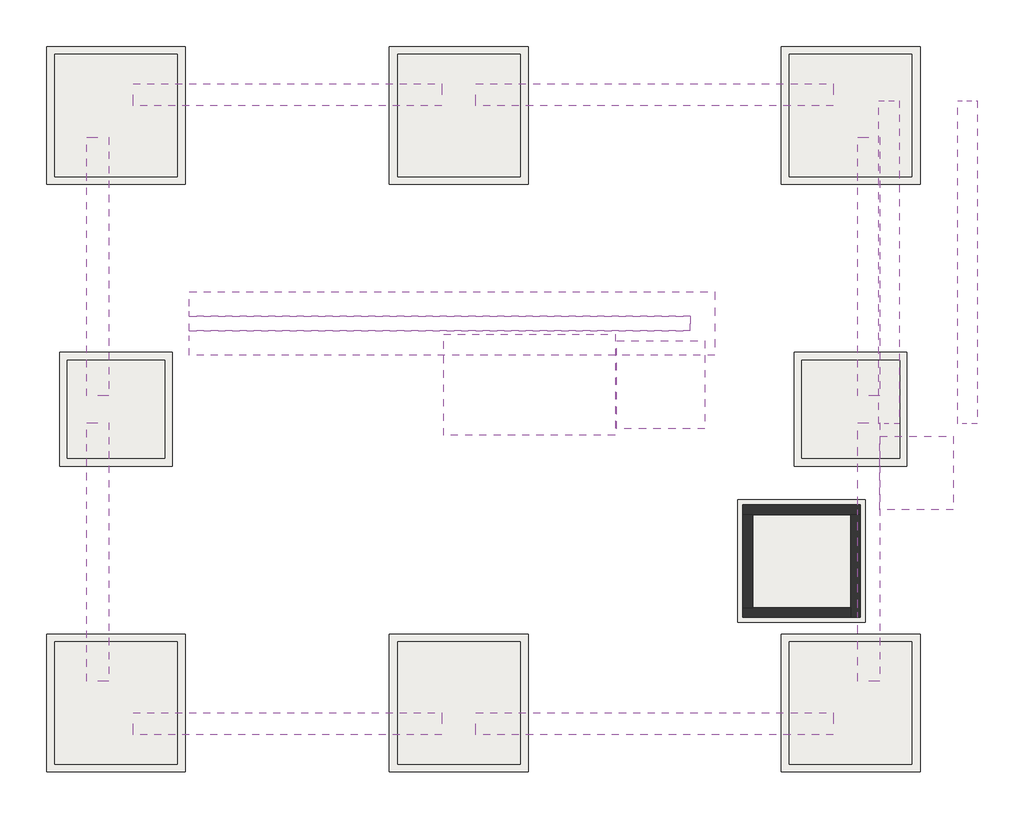
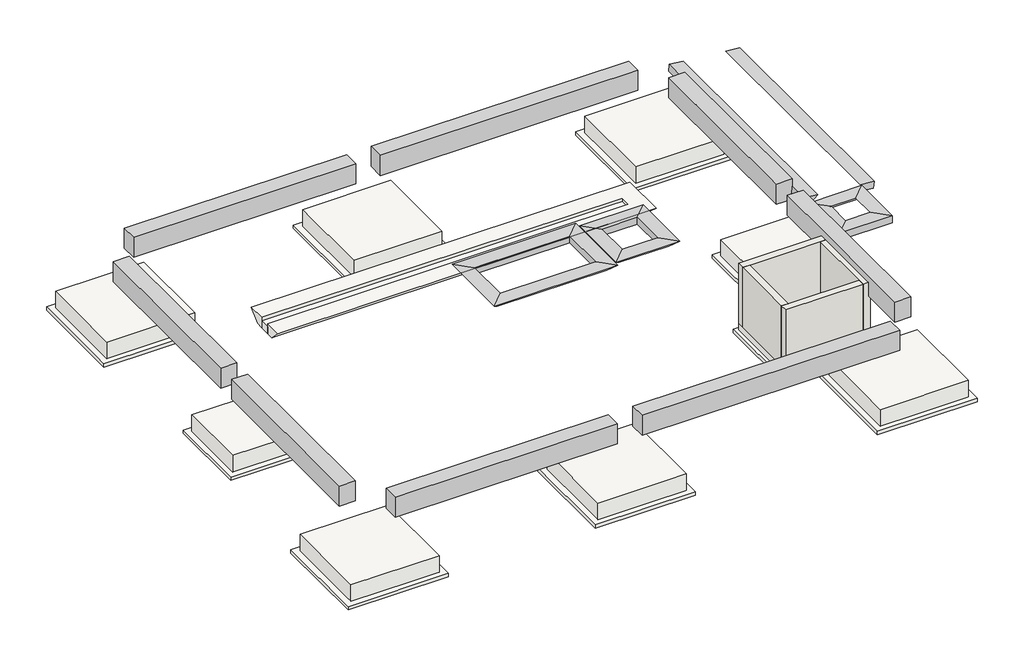
# One storey: 20 slabs, 7 beams, 5 proxies, 4 walls, 1 member.
"""IFC4 building model written with IfcOpenShell, lengths in millimetres."""

import ifcopenshell
import ifcopenshell.guid

model = None  # the IFC model being written
_history = None  # IfcOwnerHistory: only IFC2X3 demands one
_inside = {}  # id of a spatial element -> (the spatial element, [elements in it])
_under = {}  # id of a project, library or spatial element -> (it, [spatial elements below it])
_declared = {}  # id of a project -> (the project, [libraries it declares])
_typed = {}  # id of a type object -> (the type object, [elements of that type])
_made_of = {}  # id of a material, layer set ... -> (it, [elements and type objects made of it])


def new_model(schema):
    """Start an empty IFC model of exactly this schema.

    Asked for "IFC4X3", IfcOpenShell would pick the latest addendum, in which some entities
    have other attributes; the version numbers below select the first issue.
    IFC2X3 requires an IfcOwnerHistory on every rooted entity: one is made here for all.
    """
    global model, _history
    if schema == "IFC4X3":
        model = ifcopenshell.file(schema_version=(4, 3, 0, 0))
    else:
        model = ifcopenshell.file(schema=schema)
    _inside.clear()
    _under.clear()
    _declared.clear()
    _typed.clear()
    _made_of.clear()
    _history = None
    if model.schema == "IFC2X3":
        org = make("IfcOrganization", Name="unknown")
        user = make(
            "IfcPersonAndOrganization",
            ThePerson=make("IfcPerson", FamilyName="unknown"),
            TheOrganization=org,
        )
        app = make(
            "IfcApplication",
            ApplicationDeveloper=org,
            Version="unknown",
            ApplicationFullName="unknown",
            ApplicationIdentifier="unknown",
        )
        _history = make(
            "IfcOwnerHistory",
            OwningUser=user,
            OwningApplication=app,
            ChangeAction="ADDED",
            CreationDate=0,
        )
    return model


def make(cls, **values):
    """One entity of the class cls with the attributes given. An attribute that is None is left unset."""
    return model.create_entity(
        cls, **{name: value for name, value in values.items() if value is not None}
    )


def rooted(cls, **values):
    """An entity with a GlobalId (a new one), such as an element, a storey or a relation."""
    return make(cls, GlobalId=ifcopenshell.guid.new(), OwnerHistory=_history, **values)


def si_unit(unit_type, name, prefix=None):
    """IfcSIUnit, for example si_unit("LENGTHUNIT", "METRE", prefix="MILLI")."""
    return make("IfcSIUnit", UnitType=unit_type, Prefix=prefix, Name=name)


def assignment(units):
    """IfcUnitAssignment: the units of a project."""
    return None if units is None else make("IfcUnitAssignment", Units=units)


def point(xyz):
    """IfcCartesianPoint."""
    return None if xyz is None else make("IfcCartesianPoint", Coordinates=xyz)


def direction(xyz):
    """IfcDirection."""
    return None if xyz is None else make("IfcDirection", DirectionRatios=xyz)


def frame(location, z_axis=None, x_axis=None):
    """IfcAxis2Placement3D, a coordinate frame: its origin and axes. An axis left out is left unset."""
    return make(
        "IfcAxis2Placement3D",
        Location=point(location),
        Axis=direction(z_axis),
        RefDirection=direction(x_axis),
    )


def origin():
    """The frame at (0, 0, 0) with its axes left unset."""
    return frame((0.0, 0.0, 0.0))


def place(relative_to, where):
    """IfcLocalPlacement: puts the frame where relative to a parent placement (None: the world)."""
    return make(
        "IfcLocalPlacement", PlacementRelTo=relative_to, RelativePlacement=where
    )


def context(
    kind, dimensions, precision=None, world=None, true_north=None, identifier=None
):
    """IfcGeometricRepresentationContext, for example the 3D "Model" context."""
    return make(
        "IfcGeometricRepresentationContext",
        ContextIdentifier=identifier,
        ContextType=kind,
        CoordinateSpaceDimension=dimensions,
        Precision=precision,
        WorldCoordinateSystem=world,
        TrueNorth=true_north,
    )


def project(units=None, contexts=None):
    """IfcProject with its units and contexts."""
    return rooted(
        "IfcProject",
        Name="project",
        RepresentationContexts=contexts,
        UnitsInContext=assignment(units),
    )


def spatial(cls, under=None, at=None, **own):
    """A site, building, storey or space (cls), placed at a placement, below another one or the project."""
    s = rooted(cls, ObjectPlacement=at, **own)
    if under is not None:
        _under.setdefault(under.id(), (under, []))[1].append(s)
    return s


def polyline(points):
    """IfcPolyline through the points."""
    return make("IfcPolyline", Points=[point(p) for p in points])


def outline(outer, holes=None, kind="AREA"):
    """IfcArbitraryClosedProfileDef: a profile drawn as a closed curve; with holes, ...WithVoids."""
    if holes is None:
        return make("IfcArbitraryClosedProfileDef", ProfileType=kind, OuterCurve=outer)
    return make(
        "IfcArbitraryProfileDefWithVoids",
        ProfileType=kind,
        OuterCurve=outer,
        InnerCurves=holes,
    )


def extrude(swept, where, along, depth):
    """IfcExtrudedAreaSolid: the profile swept, set in the frame where, extruded along a direction by depth."""
    return make(
        "IfcExtrudedAreaSolid",
        SweptArea=swept,
        Position=where,
        ExtrudedDirection=direction(along),
        Depth=depth,
    )


def faces_of(points, faces, orient=None, outer=None):
    """IfcFace entities. A face is a list of loops; a loop is a list of indices into points, from 0.

    orient and outer hold one flag for each loop. By default every Orientation is true, the
    first loop of a face is its IfcFaceOuterBound and the others are IfcFaceBound.
    """
    made = []
    for i, loops in enumerate(faces):
        bounds = []
        for j, loop in enumerate(loops):
            is_outer = j == 0 if outer is None else outer[i][j]
            bounds.append(
                make(
                    "IfcFaceOuterBound" if is_outer else "IfcFaceBound",
                    Bound=make("IfcPolyLoop", Polygon=[points[k] for k in loop]),
                    Orientation=True if orient is None else orient[i][j],
                )
            )
        made.append(make("IfcFace", Bounds=bounds))
    return made


def faceted_brep(points, faces, orient=None, outer=None, voids=None):
    """IfcFacetedBrep: a solid bounded by flat faces; with voids (closed shells), ...WithVoids."""
    shared = [point(p) for p in points]
    hull = make("IfcClosedShell", CfsFaces=faces_of(shared, faces, orient, outer))
    if voids is None:
        return make("IfcFacetedBrep", Outer=hull)
    return make(
        "IfcFacetedBrepWithVoids",
        Outer=hull,
        Voids=[
            make(cls, CfsFaces=faces_of(shared, fs, o, b)) for cls, fs, o, b in voids
        ],
    )


def shape(context_of_items, identifier, shape_type, items):
    """IfcShapeRepresentation: the items that make up one representation, for example the "Body"."""
    return make(
        "IfcShapeRepresentation",
        ContextOfItems=context_of_items,
        RepresentationIdentifier=identifier,
        RepresentationType=shape_type,
        Items=items,
    )


def source(mapping_origin, context_of_items, identifier, shape_type, items):
    """IfcRepresentationMap: a shape defined once, which mapped items show again and again."""
    return make(
        "IfcRepresentationMap",
        MappingOrigin=mapping_origin,
        MappedRepresentation=shape(context_of_items, identifier, shape_type, items),
    )


def transform(
    local_origin,
    x_axis=None,
    y_axis=None,
    z_axis=None,
    scale=None,
    scale2=None,
    scale3=None,
    uniform=True,
):
    """IfcCartesianTransformationOperator3D, or its non-uniform kind. x_axis, y_axis, z_axis: its Axis1, 2, 3."""
    if uniform:
        return make(
            "IfcCartesianTransformationOperator3D",
            Axis1=direction(x_axis),
            Axis2=direction(y_axis),
            LocalOrigin=point(local_origin),
            Scale=scale,
            Axis3=direction(z_axis),
        )
    return make(
        "IfcCartesianTransformationOperator3DnonUniform",
        Axis1=direction(x_axis),
        Axis2=direction(y_axis),
        LocalOrigin=point(local_origin),
        Scale=scale,
        Axis3=direction(z_axis),
        Scale2=scale2,
        Scale3=scale3,
    )


def mapped(mapping_source, mapping_target):
    """IfcMappedItem: shows the shape of a source again, moved by a transform."""
    return make(
        "IfcMappedItem", MappingSource=mapping_source, MappingTarget=mapping_target
    )


def made_of(thing, what):
    """Note that an element or type object is made of a material, layer set ...; save() writes the relation."""
    if what is not None:
        _made_of.setdefault(what.id(), (what, []))[1].append(thing)
    return thing


def element(
    cls,
    number,
    at=None,
    inside=None,
    cuts=None,
    type_object=None,
    material=None,
    context=None,
    identifier="Body",
    shape_type=None,
    held_by="IfcProductDefinitionShape",
    body=None,
    shapes=None,
    **own,
):
    """One element of the class cls, such as IfcWall. Its Tag is "e" and its number.

    at: its placement. inside: the storey or other place that contains it. cuts: it is an
    opening in that element (IfcRelVoidsElement). A single representation is given by context,
    identifier, shape_type and body (its items); several are given by shapes. held_by: the class
    of the entity that holds the representations. save() writes the other relations.
    """
    e = rooted(cls, Tag="e%d" % number, ObjectPlacement=at, **own)
    if body is not None:
        shapes = [shape(context, identifier, shape_type, body)]
    if shapes is not None:
        e.Representation = make(held_by, Representations=shapes)
    if inside is not None:
        _inside.setdefault(inside.id(), (inside, []))[1].append(e)
    if cuts is not None:
        rooted(
            "IfcRelVoidsElement", RelatingBuildingElement=cuts, RelatedOpeningElement=e
        )
    if type_object is not None:
        _typed.setdefault(type_object.id(), (type_object, []))[1].append(e)
    return made_of(e, material)


def aggregate(whole, parts):
    """IfcRelAggregates: a whole, such as a stair, and the parts it consists of."""
    return rooted("IfcRelAggregates", RelatingObject=whole, RelatedObjects=parts)


def save(model, path):
    """Write the relations noted so far, then the file.

    IfcRelAggregates (storeys below a building ...), IfcRelContainedInSpatialStructure (elements
    in a storey), IfcRelDefinesByType, IfcRelAssociatesMaterial and IfcRelDeclares: one each for
    every whole, place, type object, material and project.
    """
    for whole, parts in _under.values():
        aggregate(whole, parts)
    for where, things in _inside.values():
        rooted(
            "IfcRelContainedInSpatialStructure",
            RelatedElements=things,
            RelatingStructure=where,
        )
    for kind, things in _typed.values():
        rooted("IfcRelDefinesByType", RelatedObjects=things, RelatingType=kind)
    for what, things in _made_of.values():
        rooted("IfcRelAssociatesMaterial", RelatedObjects=things, RelatingMaterial=what)
    for by, libraries in _declared.values():
        rooted("IfcRelDeclares", RelatingContext=by, RelatedDefinitions=libraries)
    model.write(path)


def slab_cd841ba3(model_context):
    return source(origin(), model_context, "Body", "Brep", [
        faceted_brep([(100.0, 18494.5382614, -200.0), (100.0, 18994.5382614, -200.0), (100.0, 18694.5382614, -500.0), (100.0, 18494.5382614, -500.0), (100.0, 18494.5382614, -300.0), (10325.0, 18494.5382614, -500.0), (10325.0, 18494.5382614, -300.0), (10325.0, 18494.5382614, -200.0), (10325.0, 18194.5382614, -200.0), (100.0, 18194.5382614, -200.0), (100.0, 17694.5382614, -200.0), (10825.0, 17694.5382614, -200.0), (10825.0, 18994.5382614, -200.0), (10525.0, 18694.5382614, -500.0), (10525.0, 17994.5382614, -500.0), (100.0, 17994.5382614, -500.0), (100.0, 18194.5382614, -500.0), (10325.0, 18194.5382614, -500.0), (10325.0, 18194.5382614, -300.0), (100.0, 18194.5382614, -300.0)], [[[0, 1, 2, 3, 4]], [[3, 5, 6, 7, 0, 4]], [[1, 0, 7, 8, 9, 10, 11, 12]], [[2, 1, 12, 13]], [[3, 2, 13, 14, 15, 16, 17, 5]], [[8, 7, 6, 5, 17, 18]], [[13, 12, 11, 14]], [[10, 9, 19, 16, 15]], [[9, 8, 18, 17, 16, 19]], [[15, 14, 11, 10]]]),
    ])


def slab_e6aba4ee(model_context):
    return source(origin(), model_context, "Body", "SweptSolid", [
        extrude(outline(polyline([(100.0, 18194.5382614), (100.0, 18494.5382614), (10325.0, 18494.5382614), (10325.0, 18194.5382614), (100.0, 18194.5382614)])), frame((0.0, 0.0, -500.0), z_axis=(0.0, 0.0, 1.0), x_axis=(1.0, 0.0, 0.0)), (0.0, 0.0, 1.0), 200.0),
    ])


def ft112_footing_rectangular_ft112_2000x2000x500_8ee35437(model_context):
    return source(origin(), model_context, "Body", "SweptSolid", [
        extrude(outline(polyline([(1000.0, 1000.0), (1000.0, -1000.0), (-1000.0, -1000.0), (-1000.0, 1000.0), (1000.0, 1000.0)])), frame((0.0, 0.0, -500.0), z_axis=(0.0, 0.0, 1.0), x_axis=(1.0, 0.0, 0.0)), (0.0, 0.0, 1.0), 500.0),
    ])


def ft112_footing_rectangular_ft112_2500x2500x500_513089b3(model_context):
    return source(origin(), model_context, "Body", "SweptSolid", [
        extrude(outline(polyline([(1250.0, 1250.0), (1250.0, -1250.0), (-1250.0, -1250.0), (-1250.0, 1250.0), (1250.0, 1250.0)])), frame((0.0, 0.0, -500.0), z_axis=(0.0, 0.0, 1.0), x_axis=(1.0, 0.0, 0.0)), (0.0, 0.0, 1.0), 500.0),
    ])


model = new_model("IFC4")

# Units and contexts
model_context = context("Model", 3, world=origin())
ifc_project = project(units=[si_unit("LENGTHUNIT", "METRE", prefix="MILLI")], contexts=[model_context])

# Site, building, storey
site = spatial("IfcSite", under=ifc_project)
building = spatial("IfcBuilding", under=site)
storey = spatial("IfcBuildingStorey", under=building, Name="1.B.O.F (FL -2200)", Elevation=-2200.0)

# Beams
placement = place(None, origin())
element("IfcBeam", 1, ObjectType="Concrete-Rectangular-Beam : BM112_450x600_UG", at=placement, inside=storey, context=model_context, shape_type="Brep", body=[
    faceted_brep([(13250.0, 9944.5382614, 0.0), (13250.0, 10394.5382614, 0.0), (5950.0, 10394.5382614, 0.0), (5950.0, 9944.5382614, 0.0), (13250.0, 9944.5382614, -600.0), (5950.0, 9944.5382614, -600.0), (13250.0, 10394.5382614, -600.0), (5950.0, 10394.5382614, -600.0), (13250.0, 10394.5382614, -200.0), (5950.0, 10394.5382614, -200.0)], [[[0, 1, 2, 3]], [[4, 0, 3, 5]], [[6, 4, 5, 7]], [[1, 8, 6, 7, 9, 2]], [[2, 9, 7, 5, 3]], [[1, 0, 4, 6, 8]]]),
])
element("IfcBeam", 2, ObjectType="Concrete-Rectangular-Beam : BM112_450x600_UG", at=placement, inside=storey, context=model_context, shape_type="Brep", body=[
    faceted_brep([(13750.0, 16319.5382614, 0.0), (13750.0, 14444.5382614, 0.0), (13750.0, 12544.5382614, 0.0), (13750.0, 11044.5382614, 0.0), (14200.0, 11044.5382614, 0.0), (14200.0, 16319.5382614, 0.0), (14200.0, 11044.5382614, -600.0), (14200.0, 16319.5382614, -600.0), (13750.0, 11044.5382614, -600.0), (13750.0, 12344.5382614, -600.0), (13800.0, 12344.5382614, -600.0), (13800.0, 14644.5382614, -600.0), (13750.0, 14644.5382614, -600.0), (13750.0, 16319.5382614, -600.0), (13750.0, 16319.5382614, -200.0), (13750.0, 14644.5382614, -200.0), (13750.0, 14444.5382614, -200.0), (13750.0, 12544.5382614, -200.0), (13750.0, 12344.5382614, -200.0), (13750.0, 11044.5382614, -200.0), (13800.0, 14644.5382614, -200.0), (13800.0, 12344.5382614, -200.0), (13800.0, 14444.5382614, -200.0)], [[[0, 1, 2, 3, 4, 5]], [[5, 4, 6, 7]], [[7, 6, 8, 9, 10, 11, 12, 13]], [[3, 2, 1, 0, 14, 13, 12, 15, 16, 17, 18, 9, 8, 19]], [[11, 20, 15, 12]], [[21, 18, 17, 16, 15, 20, 22]], [[21, 22, 20, 11, 10]], [[21, 10, 9, 18]], [[3, 19, 8, 6, 4]], [[0, 5, 7, 13, 14]]]),
])
element("IfcBeam", 3, ObjectType="Concrete-Rectangular-Beam : BM112_450x600_UG", at=placement, inside=storey, context=model_context, shape_type="Brep", body=[
    faceted_brep([(14200.0, 22144.5382614, 0.0), (13750.0, 22144.5382614, 0.0), (13750.0, 16869.5382614, 0.0), (14200.0, 16869.5382614, 0.0), (14200.0, 22144.5382614, -600.0), (14200.0, 16869.5382614, -600.0), (13750.0, 22144.5382614, -600.0), (13750.0, 16869.5382614, -600.0), (13750.0, 22144.5382614, -200.0), (13750.0, 16869.5382614, -200.0)], [[[0, 1, 2, 3]], [[4, 0, 3, 5]], [[6, 4, 5, 7]], [[1, 8, 6, 7, 9, 2]], [[1, 0, 4, 6, 8]], [[3, 2, 9, 7, 5]]]),
])
element("IfcBeam", 4, ObjectType="Concrete-Rectangular-Beam : BM112_450x600_UG", at=placement, inside=storey, context=model_context, shape_type="Brep", body=[
    faceted_brep([(5950.0, 23244.5382614, 0.0), (5950.0, 22794.5382614, 0.0), (13250.0, 22794.5382614, 0.0), (13250.0, 23244.5382614, 0.0), (5950.0, 23244.5382614, -600.0), (13250.0, 23244.5382614, -600.0), (5950.0, 22794.5382614, -600.0), (13250.0, 22794.5382614, -600.0), (5950.0, 22794.5382614, -200.0), (13250.0, 22794.5382614, -200.0)], [[[0, 1, 2, 3]], [[4, 0, 3, 5]], [[6, 4, 5, 7]], [[1, 8, 6, 7, 9, 2]], [[1, 0, 4, 6, 8]], [[3, 2, 9, 7, 5]]]),
])
element("IfcBeam", 5, ObjectType="Concrete-Rectangular-Beam : BM112_450x600_UG", at=placement, inside=storey, context=model_context, shape_type="Brep", body=[
    faceted_brep([(5250.0, 22794.5382614, 0.0), (5250.0, 23244.5382614, 0.0), (-1050.0, 23244.5382614, 0.0), (-1050.0, 22794.5382614, 0.0), (5250.0, 23244.5382614, -600.0), (-1050.0, 23244.5382614, -600.0), (5250.0, 22794.5382614, -600.0), (-1050.0, 22794.5382614, -600.0), (5250.0, 22794.5382614, -200.0), (-1050.0, 22794.5382614, -200.0)], [[[0, 1, 2, 3]], [[1, 4, 5, 2]], [[4, 6, 7, 5]], [[6, 8, 0, 3, 9, 7]], [[1, 0, 8, 6, 4]], [[3, 2, 5, 7, 9]]]),
])
element("IfcBeam", 6, ObjectType="Concrete-Rectangular-Beam : BM112_450x600_UG", at=placement, inside=storey, context=model_context, shape_type="Brep", body=[
    faceted_brep([(-1550.0, 22144.5382614, 0.0), (-2000.0, 22144.5382614, 0.0), (-2000.0, 16869.5382614, 0.0), (-1550.0, 16869.5382614, 0.0), (-2000.0, 22144.5382614, -600.0), (-2000.0, 16869.5382614, -600.0), (-1550.0, 22144.5382614, -600.0), (-1550.0, 16869.5382614, -600.0), (-1550.0, 22144.5382614, -200.0), (-1550.0, 16869.5382614, -200.0)], [[[0, 1, 2, 3]], [[1, 4, 5, 2]], [[4, 6, 7, 5]], [[6, 8, 0, 3, 9, 7]], [[1, 0, 8, 6, 4]], [[3, 2, 5, 7, 9]]]),
])
element("IfcBeam", 7, ObjectType="Concrete-Rectangular-Beam : BM112_450x600_UG", at=placement, inside=storey, context=model_context, shape_type="Brep", body=[
    faceted_brep([(-2000.0, 11044.5382614, 0.0), (-1550.0, 11044.5382614, 0.0), (-1550.0, 16319.5382614, 0.0), (-2000.0, 16319.5382614, 0.0), (-2000.0, 11044.5382614, -600.0), (-2000.0, 16319.5382614, -600.0), (-1550.0, 11044.5382614, -600.0), (-1550.0, 16319.5382614, -600.0), (-1550.0, 11044.5382614, -200.0), (-1550.0, 16319.5382614, -200.0)], [[[0, 1, 2, 3]], [[4, 0, 3, 5]], [[6, 4, 5, 7]], [[1, 8, 6, 7, 9, 2]], [[1, 0, 4, 6, 8]], [[3, 2, 9, 7, 5]]]),
])

# Proxies
element("IfcBuildingElementProxy", 8, Name="Slab Edge", ObjectType="Slab Edge", at=placement, inside=storey, context=model_context, shape_type="Brep", body=[
    faceted_brep([(8390.0, 16459.5382614, -200.0), (8390.0, 16459.5382614, -400.0), (5690.0, 16459.5382614, -400.0), (5690.0, 16459.5382614, -200.0), (8790.0, 16059.5382614, -200.0), (5290.0, 16059.5382614, -200.0), (8590.0, 16259.5382614, -400.0), (5490.0, 16259.5382614, -400.0), (8390.0, 17729.5382614, -200.0), (8390.0, 17729.5382614, -400.0), (8790.0, 18129.5382614, -200.0), (8590.0, 17929.5382614, -400.0), (5690.0, 17729.5382614, -200.0), (5690.0, 17729.5382614, -400.0), (5290.0, 18129.5382614, -200.0), (5490.0, 17929.5382614, -400.0)], [[[0, 1, 2, 3]], [[4, 0, 3, 5]], [[6, 4, 5, 7]], [[1, 6, 7, 2]], [[8, 9, 1, 0]], [[10, 8, 0, 4]], [[11, 10, 4, 6]], [[9, 11, 6, 1]], [[12, 13, 9, 8]], [[14, 12, 8, 10]], [[15, 14, 10, 11]], [[13, 15, 11, 9]], [[3, 2, 13, 12]], [[5, 3, 12, 14]], [[7, 5, 14, 15]], [[2, 7, 15, 13]]]),
])
element("IfcBuildingElementProxy", 9, Name="Slab Edge", ObjectType="Slab Edge", at=placement, inside=storey, context=model_context, shape_type="Brep", body=[
    faceted_brep([(10225.0, 16594.5382614, -200.0), (10225.0, 16594.5382614, -400.0), (9225.0, 16594.5382614, -400.0), (9225.0, 16594.5382614, -200.0), (10625.0, 16194.5382614, -200.0), (8825.0, 16194.5382614, -200.0), (10425.0, 16394.5382614, -400.0), (9025.0, 16394.5382614, -400.0), (10225.0, 17594.5382614, -200.0), (10225.0, 17594.5382614, -400.0), (10625.0, 17994.5382614, -200.0), (10425.0, 17794.5382614, -400.0), (9225.0, 17594.5382614, -200.0), (9225.0, 17594.5382614, -400.0), (8825.0, 17994.5382614, -200.0), (9025.0, 17794.5382614, -400.0)], [[[0, 1, 2, 3]], [[4, 0, 3, 5]], [[6, 4, 5, 7]], [[1, 6, 7, 2]], [[8, 9, 1, 0]], [[10, 8, 0, 4]], [[11, 10, 4, 6]], [[9, 11, 6, 1]], [[12, 13, 9, 8]], [[14, 12, 8, 10]], [[15, 14, 10, 11]], [[13, 15, 11, 9]], [[3, 2, 13, 12]], [[5, 3, 12, 14]], [[7, 5, 14, 15]], [[2, 7, 15, 13]]]),
])
element("IfcBuildingElementProxy", 10, Name="Slab Edge", ObjectType="Slab Edge", at=placement, inside=storey, context=model_context, shape_type="SweptSolid", body=[
    extrude(outline(polyline([(-620.0141724, 16171.1013164), (-421.0065284, 16191.0), (-381.2091611, 15792.9847119), (-600.1154888, 15972.0936723), (-620.0141724, 16171.1013164)])), frame((0.0, 16294.5382614, 0.0), z_axis=(0.0, 1.0, 0.0), x_axis=(0.0, 0.0, 1.0)), (0.0, 0.0, 1.0), 6600.0),
])
element("IfcBuildingElementProxy", 11, Name="Slab Edge", ObjectType="Slab Edge", at=placement, inside=storey, context=model_context, shape_type="SweptSolid", body=[
    extrude(outline(polyline([(-420.0141724, 14180.1013164), (-439.9128561, 14379.1089604), (-260.8038956, 14598.0152881), (-221.0065284, 14200.0), (-420.0141724, 14180.1013164)])), frame((0.0, 16294.5382614, 0.0), z_axis=(0.0, 1.0, 0.0), x_axis=(0.0, 0.0, 1.0)), (0.0, 0.0, 1.0), 6600.0),
])
element("IfcBuildingElementProxy", 12, Name="Slab Edge", ObjectType="Slab Edge", at=placement, inside=storey, context=model_context, shape_type="Brep", body=[
    faceted_brep([(14200.0, 16044.5382614, -220.0), (14200.0, 16044.5382614, -420.0), (14200.0, 14544.5382614, -420.0), (14200.0, 14544.5382614, -220.0), (14600.0, 15644.5382614, -220.0), (14600.0, 14944.5382614, -220.0), (14400.0, 15844.5382614, -420.0), (14400.0, 14744.5382614, -420.0), (15700.0, 14544.5382614, -420.0), (15700.0, 14544.5382614, -220.0), (15300.0, 14944.5382614, -220.0), (15500.0, 14744.5382614, -420.0), (15700.0, 16044.5382614, -420.0), (15700.0, 16044.5382614, -220.0), (15300.0, 15644.5382614, -220.0), (15500.0, 15844.5382614, -420.0)], [[[0, 1, 2, 3]], [[4, 0, 3, 5]], [[6, 4, 5, 7]], [[1, 6, 7, 2]], [[3, 2, 8, 9]], [[5, 3, 9, 10]], [[7, 5, 10, 11]], [[2, 7, 11, 8]], [[9, 8, 12, 13]], [[10, 9, 13, 14]], [[11, 10, 14, 15]], [[8, 11, 15, 12]], [[13, 12, 1, 0]], [[14, 13, 0, 4]], [[15, 14, 4, 6]], [[12, 15, 6, 1]]]),
])

# Member
element("IfcMember", 13, ObjectType="Concrete-Rectangular-Beam : BM112_450x600_UG", at=placement, inside=storey, context=model_context, shape_type="Brep", body=[
    faceted_brep([(5250.0, 9944.5382614, 0.0), (5250.0, 10394.5382614, 0.0), (-1050.0, 10394.5382614, 0.0), (-1050.0, 9944.5382614, 0.0), (5250.0, 9944.5382614, -600.0), (-1050.0, 9944.5382614, -600.0), (5250.0, 10394.5382614, -600.0), (-1050.0, 10394.5382614, -600.0), (5250.0, 10394.5382614, -200.0), (-1050.0, 10394.5382614, -200.0)], [[[0, 1, 2, 3]], [[4, 0, 3, 5]], [[6, 4, 5, 7]], [[1, 8, 6, 7, 9, 2]], [[2, 9, 7, 5, 3]], [[1, 0, 4, 6, 8]]]),
])

# Slabs
element("IfcSlab", 14, ObjectType="SL101_Lean Floor_100", at=placement, inside=storey, context=model_context, shape_type="SweptSolid", body=[
    extrude(outline(polyline([(18.583556, 12001.1722664), (18.583556, 9187.9042565), (-2818.583556, 9187.9042565), (-2818.583556, 12001.1722664), (18.583556, 12001.1722664)])), frame((0.0, 0.0, -2300.0), z_axis=(0.0, 0.0, 1.0), x_axis=(1.0, 0.0, 0.0)), (0.0, 0.0, 1.0), 100.0),
])
element("IfcSlab", 15, ObjectType="SL101_Lean Floor_100", at=placement, inside=storey, context=model_context, shape_type="SweptSolid", body=[
    extrude(outline(polyline([(7018.583556, 12001.1722664), (7018.583556, 9187.9042565), (4181.416444, 9187.9042565), (4181.416444, 12001.1722664), (7018.583556, 12001.1722664)])), frame((0.0, 0.0, -2300.0), z_axis=(0.0, 0.0, 1.0), x_axis=(1.0, 0.0, 0.0)), (0.0, 0.0, 1.0), 100.0),
])
element("IfcSlab", 16, ObjectType="SL101_Lean Floor_100", at=placement, inside=storey, context=model_context, shape_type="SweptSolid", body=[
    extrude(outline(polyline([(15018.583556, 12001.1722664), (15018.583556, 9187.9042565), (12181.416444, 9187.9042565), (12181.416444, 12001.1722664), (15018.583556, 12001.1722664)])), frame((0.0, 0.0, -2300.0), z_axis=(0.0, 0.0, 1.0), x_axis=(1.0, 0.0, 0.0)), (0.0, 0.0, 1.0), 100.0),
])
element("IfcSlab", 17, ObjectType="SL101_Lean Floor_100", at=placement, inside=storey, context=model_context, shape_type="SweptSolid", body=[
    extrude(outline(polyline([(18.583556, 24001.1722664), (18.583556, 21187.9042565), (-2818.583556, 21187.9042565), (-2818.583556, 24001.1722664), (18.583556, 24001.1722664)])), frame((0.0, 0.0, -2300.0), z_axis=(0.0, 0.0, 1.0), x_axis=(1.0, 0.0, 0.0)), (0.0, 0.0, 1.0), 100.0),
])
element("IfcSlab", 18, ObjectType="SL101_Lean Floor_100", at=placement, inside=storey, context=model_context, shape_type="SweptSolid", body=[
    extrude(outline(polyline([(7018.583556, 24001.1722664), (7018.583556, 21187.9042565), (4181.416444, 21187.9042565), (4181.416444, 24001.1722664), (7018.583556, 24001.1722664)])), frame((0.0, 0.0, -2300.0), z_axis=(0.0, 0.0, 1.0), x_axis=(1.0, 0.0, 0.0)), (0.0, 0.0, 1.0), 100.0),
])
element("IfcSlab", 19, ObjectType="SL101_Lean Floor_100", at=placement, inside=storey, context=model_context, shape_type="SweptSolid", body=[
    extrude(outline(polyline([(15018.583556, 24001.1722664), (15018.583556, 21187.9042565), (12181.416444, 21187.9042565), (12181.416444, 24001.1722664), (15018.583556, 24001.1722664)])), frame((0.0, 0.0, -2300.0), z_axis=(0.0, 0.0, 1.0), x_axis=(1.0, 0.0, 0.0)), (0.0, 0.0, 1.0), 100.0),
])
element("IfcSlab", 20, ObjectType="SL101_Lean Floor_100", at=placement, inside=storey, context=model_context, shape_type="SweptSolid", body=[
    extrude(outline(polyline([(-251.1867019, 17756.5623227), (-251.1867019, 15432.5142002), (-2548.8132981, 15432.5142002), (-2548.8132981, 17756.5623227), (-251.1867019, 17756.5623227)])), frame((0.0, 0.0, -2300.0), z_axis=(0.0, 0.0, 1.0), x_axis=(1.0, 0.0, 0.0)), (0.0, 0.0, 1.0), 100.0),
])
element("IfcSlab", 21, ObjectType="SL101_Lean Floor_100", at=placement, inside=storey, context=model_context, shape_type="SweptSolid", body=[
    extrude(outline(polyline([(14748.8132981, 17756.5623227), (14748.8132981, 15432.5142002), (12451.1867019, 15432.5142002), (12451.1867019, 17756.5623227), (14748.8132981, 17756.5623227)])), frame((0.0, 0.0, -2300.0), z_axis=(0.0, 0.0, 1.0), x_axis=(1.0, 0.0, 0.0)), (0.0, 0.0, 1.0), 100.0),
])
element("IfcSlab", 22, ObjectType="SL101_Lean Floor_100", at=placement, inside=storey, context=model_context, shape_type="SweptSolid", body=[
    extrude(outline(polyline([(13900.0, 14744.5382614), (13900.0, 12244.5382614), (11300.0, 12244.5382614), (11300.0, 14744.5382614), (13900.0, 14744.5382614)])), frame((0.0, 0.0, -2300.0), z_axis=(0.0, 0.0, 1.0), x_axis=(1.0, 0.0, 0.0)), (0.0, 0.0, 1.0), 100.0),
])
slab_shape = slab_cd841ba3(model_context)
element("IfcSlab", 23, ObjectType="Ditch Wall 1 : Ditch Wall 1", at=placement, inside=storey, context=model_context, shape_type="MappedRepresentation", body=[
    mapped(slab_shape, transform((0.0, 0.0, 0.0), x_axis=(1.0, 0.0, 0.0), y_axis=(0.0, 1.0, 0.0), z_axis=(0.0, 0.0, 1.0))),
])
slab_2_shape = slab_e6aba4ee(model_context)
element("IfcSlab", 24, ObjectType="Ditch 2 : Ditch 2", at=placement, inside=storey, context=model_context, shape_type="MappedRepresentation", body=[
    mapped(slab_2_shape, transform((0.0, 0.0, 0.0), x_axis=(1.0, 0.0, 0.0), y_axis=(0.0, 1.0, 0.0), z_axis=(0.0, 0.0, 1.0))),
])
ft112_footing_rectangular_ft112_2000x2000x500_shape = ft112_footing_rectangular_ft112_2000x2000x500_8ee35437(model_context)
element("IfcSlab", 25, ObjectType="FT112-Footing-Rectangular : FT112_2000x2000x500", at=placement, inside=storey, context=model_context, shape_type="MappedRepresentation", body=[
    mapped(ft112_footing_rectangular_ft112_2000x2000x500_shape, transform((-1400.0, 16594.5382614, -1700.0), x_axis=(1.0, 0.0, 0.0), y_axis=(0.0, 1.0, 0.0), z_axis=(0.0, 0.0, 1.0))),
])
element("IfcSlab", 26, ObjectType="FT112-Footing-Rectangular : FT112_2000x2000x500", at=placement, inside=storey, context=model_context, shape_type="MappedRepresentation", body=[
    mapped(ft112_footing_rectangular_ft112_2000x2000x500_shape, transform((13600.0, 16594.5382614, -1700.0), x_axis=(1.0, 0.0, 0.0), y_axis=(0.0, 1.0, 0.0), z_axis=(0.0, 0.0, 1.0))),
])
element("IfcSlab", 27, ObjectType="FT112-Footing-Rectangular : FT112_2500x2500x500", at=placement, inside=storey, context=model_context, shape_type="SweptSolid", body=[
    extrude(outline(polyline([(-150.0, 11844.5382614), (-150.0, 9344.5382614), (-2650.0, 9344.5382614), (-2650.0, 11844.5382614), (-150.0, 11844.5382614)])), frame((0.0, 0.0, -2200.0), z_axis=(0.0, 0.0, 1.0), x_axis=(1.0, 0.0, 0.0)), (0.0, 0.0, 1.0), 500.0),
])
ft112_footing_rectangular_ft112_2500x2500x500_shape = ft112_footing_rectangular_ft112_2500x2500x500_513089b3(model_context)
element("IfcSlab", 28, ObjectType="FT112-Footing-Rectangular : FT112_2500x2500x500", at=placement, inside=storey, context=model_context, shape_type="MappedRepresentation", body=[
    mapped(ft112_footing_rectangular_ft112_2500x2500x500_shape, transform((-1400.0, 22594.5382614, -1700.0), x_axis=(1.0, 0.0, 0.0), y_axis=(0.0, 1.0, 0.0), z_axis=(0.0, 0.0, 1.0))),
])
element("IfcSlab", 29, ObjectType="FT112-Footing-Rectangular : FT112_2500x2500x500", at=placement, inside=storey, context=model_context, shape_type="MappedRepresentation", body=[
    mapped(ft112_footing_rectangular_ft112_2500x2500x500_shape, transform((5600.0, 22594.5382614, -1700.0), x_axis=(1.0, 0.0, 0.0), y_axis=(0.0, 1.0, 0.0), z_axis=(0.0, 0.0, 1.0))),
])
element("IfcSlab", 30, ObjectType="FT112-Footing-Rectangular : FT112_2500x2500x500", at=placement, inside=storey, context=model_context, shape_type="MappedRepresentation", body=[
    mapped(ft112_footing_rectangular_ft112_2500x2500x500_shape, transform((13600.0, 22594.5382614, -1700.0), x_axis=(1.0, 0.0, 0.0), y_axis=(0.0, 1.0, 0.0), z_axis=(0.0, 0.0, 1.0))),
])
element("IfcSlab", 31, ObjectType="FT112-Footing-Rectangular : FT112_2500x2500x500", at=placement, inside=storey, context=model_context, shape_type="MappedRepresentation", body=[
    mapped(ft112_footing_rectangular_ft112_2500x2500x500_shape, transform((13600.0, 10594.5382614, -1700.0), x_axis=(1.0, 0.0, 0.0), y_axis=(0.0, 1.0, 0.0), z_axis=(0.0, 0.0, 1.0))),
])
element("IfcSlab", 32, ObjectType="FT112-Footing-Rectangular : FT112_2500x2500x500", at=placement, inside=storey, context=model_context, shape_type="MappedRepresentation", body=[
    mapped(ft112_footing_rectangular_ft112_2500x2500x500_shape, transform((5600.0, 10594.5382614, -1700.0), x_axis=(1.0, 0.0, 0.0), y_axis=(0.0, 1.0, 0.0), z_axis=(0.0, 0.0, 1.0))),
])
element("IfcSlab", 33, ObjectType="MF111_THK.200", at=placement, inside=storey, context=model_context, shape_type="SweptSolid", body=[
    extrude(outline(polyline([(13800.0, 14644.5382614), (13800.0, 12344.5382614), (11400.0, 12344.5382614), (11400.0, 14644.5382614), (13800.0, 14644.5382614)])), frame((0.0, 0.0, -2200.0), z_axis=(0.0, 0.0, 1.0), x_axis=(1.0, 0.0, 0.0)), (0.0, 0.0, 1.0), 200.0),
])

# Walls
element("IfcWall", 34, ObjectType="WA111-UG RC Wall 200mm", at=placement, inside=storey, context=model_context, shape_type="Brep", body=[
    faceted_brep([(11400.0, 14444.5382614, -2000.0), (11600.0, 14444.5382614, -2000.0), (13600.0, 14444.5382614, -2000.0), (13800.0, 14444.5382614, -2000.0), (13800.0, 14444.5382614, -200.0), (13600.0, 14444.5382614, -200.0), (11600.0, 14444.5382614, -200.0), (11400.0, 14444.5382614, -200.0), (11400.0, 14644.5382614, -2000.0), (11400.0, 14644.5382614, -200.0), (13750.0, 14644.5382614, -200.0), (13800.0, 14644.5382614, -200.0), (13800.0, 14644.5382614, -600.0), (13800.0, 14644.5382614, -2000.0)], [[[0, 1, 2, 3, 4, 5, 6, 7]], [[8, 9, 10, 11, 12, 13]], [[3, 2, 1, 0, 8, 13]], [[7, 6, 5, 4, 11, 10, 9]], [[4, 3, 13, 12, 11]], [[0, 7, 9, 8]]]),
])
element("IfcWall", 35, ObjectType="WA111-UG RC Wall 200mm", at=placement, inside=storey, context=model_context, shape_type="Brep", body=[
    faceted_brep([(13600.0, 14444.5382614, -2000.0), (13600.0, 12544.5382614, -2000.0), (13600.0, 12344.5382614, -2000.0), (13600.0, 12344.5382614, -200.0), (13600.0, 12544.5382614, -200.0), (13600.0, 14444.5382614, -200.0), (13800.0, 14444.5382614, -2000.0), (13800.0, 14444.5382614, -200.0), (13800.0, 12344.5382614, -200.0), (13800.0, 12344.5382614, -600.0), (13800.0, 12344.5382614, -2000.0), (13750.0, 12344.5382614, -200.0)], [[[0, 1, 2, 3, 4, 5]], [[6, 7, 8, 9, 10]], [[2, 1, 0, 6, 10]], [[5, 4, 3, 11, 8, 7]], [[0, 5, 7, 6]], [[3, 2, 10, 9, 8, 11]]]),
])
element("IfcWall", 36, ObjectType="WA111-UG RC Wall 200mm", at=placement, inside=storey, context=model_context, shape_type="Brep", body=[
    faceted_brep([(13600.0, 12544.5382614, -2000.0), (11600.0, 12544.5382614, -2000.0), (11400.0, 12544.5382614, -2000.0), (11400.0, 12544.5382614, -200.0), (11600.0, 12544.5382614, -200.0), (13600.0, 12544.5382614, -200.0), (13600.0, 12344.5382614, -2000.0), (13600.0, 12344.5382614, -200.0), (11400.0, 12344.5382614, -200.0), (11400.0, 12344.5382614, -2000.0)], [[[0, 1, 2, 3, 4, 5]], [[6, 7, 8, 9]], [[2, 1, 0, 6, 9]], [[5, 4, 3, 8, 7]], [[0, 5, 7, 6]], [[3, 2, 9, 8]]]),
])
element("IfcWall", 37, ObjectType="WA111-UG RC Wall 200mm", at=placement, inside=storey, context=model_context, shape_type="SweptSolid", body=[
    extrude(outline(polyline([(11600.0, 14444.5382614), (11600.0, 12544.5382614), (11400.0, 12544.5382614), (11400.0, 14444.5382614), (11600.0, 14444.5382614)])), frame((0.0, 0.0, -2000.0), z_axis=(0.0, 0.0, 1.0), x_axis=(1.0, 0.0, 0.0)), (0.0, 0.0, 1.0), 1800.0),
])

save(model, "model.ifc")

# Revit data of these elements
# Project information
#   Project ISM Data = "<?xml version=\"1.0\" encoding=\"utf-16\"?><ism schema_version=\"03.00\"><section_positioning><element family_name=\"CO_RC_REC\" symbol_name=\"CCC12_Rec_450x450\" section_id=\"F2ADF140-E21A-4820-8170-6F63D956DCAD\" category=\"OST_StructuralColumns\" mirror_y=\"0\" mirror_x=\"0\" /><element family_name=\"CO_RC_REC\" symbol_name=\"CCC12_Rec_450x450\" section_id=\"B35A310E-4F33-462b-819C-3ADD300C0CEB\" category=\"OST_StructuralColumns\" mirror_y=\"0\" mirror_x=\"0\" /><element family_name=\"CO_RC_REC\" symbol_name=\"CCC12_Rec_450x450\" section_id=\"711054EC-0DB2-46e3-AD20-004560300C00\" category=\"OST_StructuralColumns\" mirror_y=\"0\" mirror_x=\"0\" /><element family_name=\"CO_RC_REC\" symbol_name=\"300 x 450\" section_id=\"B5C54EC9-8EBD-4860-AB72-EF5791AED394\" category=\"OST_StructuralColumns\" mirror_y=\"0\" mirror_x=\"0\" /><element family_name=\"GI_RC_C\" symbol_name=\"SGC11_400x500\" section_id=\"0A7B8D02-9EA4-4aa9-A41A-E30BB5B6B6C5\" category=\"OST_StructuralFraming\" mirror_y=\"0\" mirror_x=\"0\" /><element family_name=\"GI_RC_C\" symbol_name=\"SGC11_400x500\" section_id=\"714BBD27-DB58-47da-B54C-5806291C2D3C\" category=\"OST_StructuralFraming\" mirror_y=\"0\" mirror_x=\"0\" /><element family_name=\"GI_RC_C\" symbol_name=\"SGC11_400x500\" section_id=\"F36E62C1-13EE-4807-A3C1-899E23E0BEDE\" category=\"OST_StructuralFraming\" mirror_y=\"0\" mirror_x=\"0\" /><element family_name=\"GI_RC_C\" symbol_name=\"SGC11_400x500\" section_id=\"F5448801-679E-44d6-8F46-E676344F8165\" category=\"OST_StructuralFraming\" mirror_y=\"0\" mirror_x=\"0\" /><element family_name=\"GI_RC_C\" symbol_name=\"SGC11_400x600\" section_id=\"05D74241-6318-4cac-95F5-7B878260D5B5\" category=\"OST_StructuralFraming\" mirror_y=\"0\" mirror_x=\"0\" /><element family_name=\"GI_RC_C\" symbol_name=\"SGC11_400x500\" section_id=\"846DCB0C-E06B-4978-9D43-E1CC0FDE7595\" category=\"OST_StructuralFraming\" mirror_y=\"0\" mirror_x=\"0\" /><element family_name=\"GI_RC_C\" symbol_name=\"SGC11_400x500\" section_id=\"2ADF82B8-986D-4f44-85DE-89D921292160\" category=\"OST_StructuralFraming\" mirror_y=\"0\" mirror_x=\"0\" /><element family_name=\"GI_RC_C\" symbol_name=\"SGC11_400x500\" section_id=\"7AF371ED-051B-4a30-8826-11F11C212B73\" category=\"OST_StructuralFraming\" mirror_y=\"0\" mirror_x=\"0\" /><element family_name=\"GI_RC_C\" symbol_name=\"SGC11_400x500\" section_id=\"2FE74006-ADDA-412f-A522-853919E62B4D\" category=\"OST_StructuralFraming\" mirror_y=\"0\" mirror_x=\"0\" /><element family_name=\"GI_RC_C\" symbol_name=\"SGC11_400x500\" section_id=\"09B63641-D581-4a6c-A18E-54C17EC989A4\" category=\"OST_StructuralFraming\" mirror_y=\"0\" mirror_x=\"0\" /><element family_name=\"GI_RC_C\" symbol_name=\"SGC11_400x500\" section_id=\"0DD6B52A-77D0-45a1-82B1-8236ED57078C\" category=\"OST_StructuralFraming\" mirror_y=\"0\" mirror_x=\"0\" /><element family_name=\"GI_RC_C\" symbol_name=\"SGC11_400x500\" section_id=\"35D311D2-DEB8-4469-97DE-110B6DF5B84D\" category=\"OST_StructuralFraming\" mirror_y=\"0\" mirror_x=\"0\" /><element family_name=\"GI_RC_C\" symbol_name=\"SGC11_400x500\" section_id=\"0D3CCDE5-CFF9-431b-A4BD-01BF6636D6BD\" category=\"OST_StructuralFraming\" mirror_y=\"0\" mirror_x=\"0\" /><element family_name=\"GI_RC_C\" symbol_name=\"SGC11_400x500\" section_id=\"C62B2A5B-024A-47ac-B030-C17A67E64A7B\" category=\"OST_StructuralFraming\" mirror_y=\"0\" mirror_x=\"0\" /><element family_name=\"GI_RC_C\" symbol_name=\"SGC11_400x500\" section_id=\"944C6E43-E607-48c3-8358-9E6CB88346E7\" category=\"OST_StructuralFraming\" mirror_y=\"0\" mirror_x=\"0\" /><element family_name=\"GI_RC_C\" symbol_name=\"SGC11_400x500\" section_id=\"A4B1F42D-B1C2-4ad2-8AD6-DB0D5E05998D\" category=\"OST_StructuralFraming\" mirror_y=\"0\" mirror_x=\"0\" /><element family_name=\"GI_RC_C\" symbol_name=\"SGC11_400x500\" section_id=\"007E6C70-1139-4b48-B003-C76FAD4C249A\" category=\"OST_StructuralFraming\" mirror_y=\"0\" mirror_x=\"0\" /><element family_name=\"GI_RC_C\" symbol_name=\"SGC11_400x500\" section_id=\"9941AC94-F03A-464c-9912-04590E0C31E0\" category=\"OST_StructuralFraming\" mirror_y=\"0\" mirror_x=\"0\" /><element family_name=\"GI_RC_C\" symbol_name=\"SGC11_400x500\" section_id=\"CFD98B8D-8FF4-4e71-A909-0FE7DBCE924E\" category=\"OST_StructuralFraming\" mirror_y=\"0\" mirror_x=\"0\" /><element family_name=\"GI_RC_C\" symbol_name=\"SGC11_400x500\" section_id=\"58262161-98E6-45c8-B2BD-4508105FF662\" category=\"OST_StructuralFraming\" mirror_y=\"0\" mirror_x=\"0\" /><element family_name=\"GI_RC_C\" symbol_name=\"SGC11_400x500\" section_id=\"66AB4841-610A-4883-97F7-1282A56484E1\" category=\"OST_StructuralFraming\" mirror_y=\"0\" mirror_x=\"0\" /><element family_name=\"GI_RC_C\" symbol_name=\"SGC11_400x500\" section_id=\"D2B324BE-BBD6-49da-9730-60EA7AD4D3A0\" category=\"OST_StructuralFraming\" mirror_y=\"0\" mirror_x=\"0\" /><element family_name=\"GI_RC_C\" symbol_name=\"SGC11_400x500\" section_id=\"92A8ECE7-C053-46b1-92ED-F2C041617E7B\" category=\"OST_StructuralFraming\" mirror_y=\"0\" mirror_x=\"0\" /><element family_name=\"GI_RC_C\" symbol_name=\"SGC11_400x500\" section_id=\"B4C4BDB0-65C4-4016-9C78-DBD77E229523\" category=\"OST_StructuralFraming\" mirror_y=\"0\" mirror_x=\"0\" /><element family_name=\"GI_RC_C\" symbol_name=\"SGC11_400x500\" section_id=\"57270646-162F-4c83-BDB7-A5FBEA9120BD\" category=\"OST_StructuralFraming\" mirror_y=\"0\" mirror_x=\"0\" /><element family_name=\"GI_RC_C\" symbol_name=\"SGC11_400x500\" section_id=\"BDEF733F-00AA-4eee-B6C6-50229FC1D236\" category=\"OST_StructuralFraming\" mirror_y=\"0\" mirror_x=\"0\" /><element family_name=\"GI_RC_C\" symbol_name=\"SGC11_400x500\" section_id=\"84A94E1E-3074-40f4-9690-97191755F019\" category=\"OST_StructuralFraming\" mirror_y=\"0\" mirror_x=\"0\" /><element family_name=\"GI_RC_C\" symbol_name=\"SGC11_400x500\" section_id=\"8A7D913D-7967-4718-912D-B83DF0AD2EDD\" category=\"OST_StructuralFraming\" mirror_y=\"0\" mirror_x=\"0\" /><element family_name=\"GI_RC_C\" symbol_name=\"SGC11_400x500\" section_id=\"83553D70-90FA-469c-B5C3-EF03F3FC6475\" category=\"OST_StructuralFraming\" mirror_y=\"0\" mirror_x=\"0\" /><element family_name=\"GI_RC_C\" symbol_name=\"SGC11_400x500\" section_id=\"6880C1E4-C50B-4c1b-B61C-23F2D8C46873\" category=\"OST_StructuralFraming\" mirror_y=\"0\" mirror_x=\"0\" /><element family_name=\"GI_RC_C\" symbol_name=\"SGC11_400x500\" section_id=\"08594C43-CD40-47de-A3BA-8BFB47F64994\" category=\"OST_StructuralFraming\" mirror_y=\"0\" mirror_x=\"0\" /><element family_name=\"GI_RC_C\" symbol_name=\"SGC11_400x500\" section_id=\"7D2E11FA-A5E1-4434-B9BE-AABA1A16CA03\" category=\"OST_StructuralFraming\" mirror_y=\"0\" mirror_x=\"0\" /><element family_name=\"GI_RC_C\" symbol_name=\"SGC11_400x500\" section_id=\"D892DFA4-5441-4ad2-A390-253492293B1B\" category=\"OST_StructuralFraming\" mirror_y=\"0\" mirror_x=\"0\" /><element family_name=\"GI_RC_C\" symbol_name=\"SGC11_400x500\" section_id=\"E5A32FE6-89C4-49f1-B3B9-1CABE7C48A4D\" category=\"OST_StructuralFraming\" mirror_y=\"0\" mirror_x=\"0\" /><element family_name=\"GI_RC_C\" symbol_name=\"SGC11_400x500\" section_id=\"8AE872C2-5DBE-47c5-934B-7E964A84B589\" category=\"OST_StructuralFraming\" mirror_y=\"0\" mirror_x=\"0\" /><element family_name=\"GI_RC_C\" symbol_name=\"SGC11_400x500\" section_id=\"3C847B60-488A-4604-A400-16A3A65E919B\" category=\"OST_StructuralFraming\" mirror_y=\"0\" mirror_x=\"0\" /><element family_name=\"GI_RC_C\" symbol_name=\"SGC11_400x500\" section_id=\"DBEC432A-3F7B-4266-AD99-2A937DC70BCF\" category=\"OST_StructuralFraming\" mirror_y=\"0\" mirror_x=\"0\" /><element family_name=\"GI_RC_C\" symbol_name=\"SGC11_400x500\" section_id=\"59403DD6-7A51-48aa-A3BE-962457E6F10E\" category=\"OST_StructuralFraming\" mirror_y=\"0\" mirror_x=\"0\" /><element family_name=\"GI_RC_C\" symbol_name=\"SGC11_400x500\" section_id=\"11CDDF5D-38B6-43b2-A291-FC188BE232BC\" category=\"OST_StructuralFraming\" mirror_y=\"0\" mirror_x=\"0\" /><element family_name=\"GI_RC_C\" symbol_name=\"SGC11_400x500\" section_id=\"10BF2843-EFC9-4136-933C-5B270D970277\" category=\"OST_StructuralFraming\" mirror_y=\"0\" mirror_x=\"0\" /><element family_name=\"GI_RC_C\" symbol_name=\"SGC11_400x500\" section_id=\"E1B09A9C-F6C6-47d9-976B-E313C0E3F52B\" category=\"OST_StructuralFraming\" mirror_y=\"0\" mirror_x=\"0\" /><element family_name=\"GI_RC_C\" symbol_name=\"SGC11_400x500\" section_id=\"A3A22EC3-26C8-4588-A0AB-AFAE02DF267E\" category=\"OST_StructuralFraming\" mirror_y=\"0\" mirror_x=\"0\" /><element family_name=\"GI_RC_C\" symbol_name=\"SGC11_400x500\" section_id=\"114828FC-BDC1-4343-9119-BCB5395DAA64\" category=\"OST_StructuralFraming\" mirror_y=\"0\" mirror_x=\"0\" /><element family_name=\"GI_RC_C\" symbol_name=\"SGC11_400x500\" section_id=\"797626F9-3558-4623-826F-15FB93088CB3\" category=\"OST_StructuralFraming\" mirror_y=\"0\" mirror_x=\"0\" /><element family_name=\"GI_RC_C\" symbol_name=\"SGC11_400x500\" section_id=\"4BF369CD-DF09-4346-96CB-C6C6380A2599\" category=\"OST_StructuralFraming\" mirror_y=\"0\" mirror_x=\"0\" /><element family_name=\"GI_RC_C\" symbol_name=\"SGC11_400x500\" section_id=\"722B46BA-61C4-44a1-9ECF-325B60B6688D\" category=\"OST_StructuralFraming\" mirror_y=\"0\" mirror_x=\"0\" /><element family_name=\"GI_RC_C\" symbol_name=\"SGC11_400x500\" section_id=\"C33DBE84-19C1-4379-AB6E-A41F7420F18C\" category=\"OST_StructuralFraming\" mirror_y=\"0\" mirror_x=\"0\" /><element family_name=\"GI_RC_C\" symbol_name=\"SGC11_400x500\" section_id=\"1F2D3B75-66F2-4d88-A1DD-647969477B86\" category=\"OST_StructuralFraming\" mirror_y=\"0\" mirror_x=\"0\" /><element family_name=\"GI_RC_C\" symbol_name=\"SGC11_400x500\" section_id=\"DFBF96B2-410A-4f39-80C4-D8CF78561C93\" category=\"OST_StructuralFraming\" mirror_y=\"0\" mirror_x=\"0\" /><element family_name=\"GI_RC_C\" symbol_name=\"SGC11_400x500\" section_id=\"D6793CD3-AB64-417c-9C28-8B18A0A2D336\" category=\"OST_StructuralFraming\" mirror_y=\"0\" mirror_x=\"0\" /><element family_name=\"GI_RC_C\" symbol_name=\"SGC11_400x500\" section_id=\"90884AC0-EA00-4caa-86E1-E6B886FD90ED\" category=\"OST_StructuralFraming\" mirror_y=\"0\" mirror_x=\"0\" /><element family_name=\"GI_RC_C\" symbol_name=\"SGC11_400x500\" section_id=\"64BC7B89-F7C8-4dae-A5C8-F10DF9E5F6BA\" category=\"OST_StructuralFraming\" mirror_y=\"0\" mirror_x=\"0\" /><element family_name=\"GI_RC_C\" symbol_name=\"SGC11_400x500\" section_id=\"D82E4D85-2728-40e5-9F60-1C7FB2990D78\" category=\"OST_StructuralFraming\" mirror_y=\"0\" mirror_x=\"0\" /><element family_name=\"GI_RC_C\" symbol_name=\"SGC11_400x500\" section_id=\"1E6D05B9-BF84-4669-AA27-948ADA1D511E\" category=\"OST_StructuralFraming\" mirror_y=\"0\" mirror_x=\"0\" /><element family_name=\"GI_RC_C\" symbol_name=\"SGC11_400x500\" section_id=\"73608CB2-EB94-466e-883D-814030EF49D6\" category=\"OST_StructuralFraming\" mirror_y=\"0\" mirror_x=\"0\" /><element family_name=\"GI_RC_C\" symbol_name=\"SGC11_400x500\" section_id=\"4EAF07EF-4E08-4065-9F08-BF69D4413867\" category=\"OST_StructuralFraming\" mirror_y=\"1\" mirror_x=\"1\" /></section_positioning><surface_member_mappings /><element_binding><element revit_id=\"0aa8b22b-49cd-4eb2-b994-d423f7aad482-0014435e\" ism_id=\"637A3C89-B4B9-4EE4-9E04-FF73E7A5771D\" /><element revit_id=\"af7cfdda-f71a-4a09-bb03-63e0c16d5d93-00152efa\" ism_id=\"088C1743-AFAE-4D55-B14F-2330F3A79060\" /><element revit_id=\"af7cfdda-f71a-4a09-bb03-63e0c16d5d93-00152efc\" ism_id=\"38278b30-864a-4bde-bfee-6c2d4309b281\" /><element revit_id=\"af7cfdda-f71a-4a09-bb03-63e0c16d5d93-00152eff\" ism_id=\"e2895b00-887b-4cf1-92a9-c4855f67b579\" /><element revit_id=\"af7cfdda-f71a-4a09-bb03-63e0c16d5d93-00152f02\" ism_id=\"a6b13b86-1938-47ee-8937-754844bb71d9\" /><element revit_id=\"af7cfdda-f71a-4a09-bb03-63e0c16d5d93-00152f05\" ism_id=\"b3cdb4ae-01be-49a8-8521-dfb37fcb7a09\" /><element revit_id=\"af7cfdda-f71a-4a09-bb03-63e0c16d5d93-00152f08\" ism_id=\"0a200294-2d0f-43b2-a10b-c345be42008c\" /><element revit_id=\"af7cfdda-f71a-4a09-bb03-63e0c16d5d
